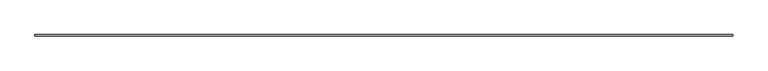
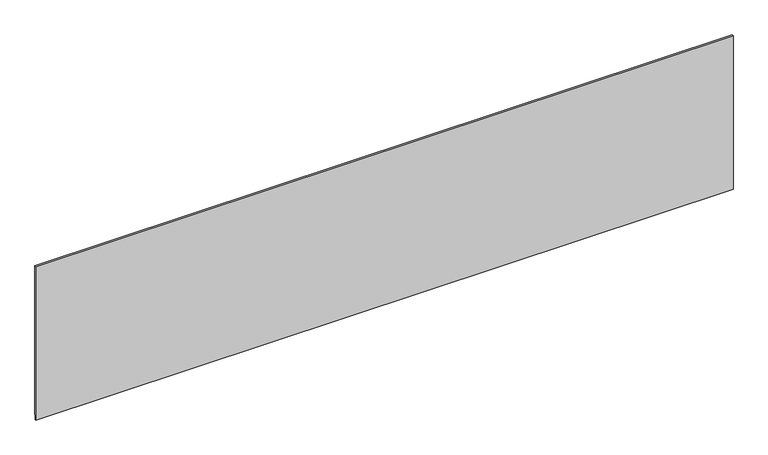
"""IFC4 building model written with IfcOpenShell, lengths in millimetres: proxy geometry, Generic Models 7:Generic Models 1:5:Generic Models 1:5 : Generic Models 7:Generic Models 1:337419:34 : Generic Models 7:Generic Models 1:5:Generic Models 1:5 : Generic Models 7:Generic Models 1:337419:311462."""

from ifc_helpers import new_model, si_unit, frame, origin, place, context, project, spatial, polyline, outline, extrude, source, transform, mapped, element, save


def generic_models_37c5037e(model_context):
    return source(origin(), model_context, "Body", "SweptSolid", [
        extrude(outline(polyline([(-579029.0720892, 3723.834699), (-579038.7913841, 3723.834699), (-579038.7913841, 6155.090949), (-579019.7413841, 6155.090949), (-579019.7413841, 3795.8780043), (-579029.0720892, 3784.758103), (-579029.0720892, 3723.834699)])), frame((793360.8632437, 0.0, 0.0), z_axis=(1.0, 0.0, 0.0), x_axis=(0.0, 1.0, 0.0)), (0.0, 0.0, 1.0), 10450.5125),
    ])


if __name__ == "__main__":
    model = new_model("IFC4")
    model_context = context("Model", 3, world=origin())
    ifc_project = project(units=[si_unit("LENGTHUNIT", "METRE", prefix="MILLI")], contexts=[model_context])
    site = spatial("IfcSite", under=ifc_project)
    building = spatial("IfcBuilding", under=site)
    placement = place(None, origin())
    generic_models_shape = generic_models_37c5037e(model_context)
    element("IfcBuildingElementProxy", 1, Name="Generic Models 7:Generic Models 1:5:Generic Models 1:5 : Generic Models 7:Generic Models 1:337419:34 : Generic Models 7:Generic Models 1:5:Generic Models 1:5 : Generic Models 7:Generic Models 1:337419:311462", ObjectType="Generic Models 7:Generic Models 1:5:Generic Models 1:5 : Generic Models 7:Generic Models 1:337419:34 : Generic Models 7:Generic Models 1:5:Generic Models 1:5 : Generic Models 7:Generic Models 1:337419:311462", at=placement, inside=building, context=model_context, shape_type="MappedRepresentation", body=[
        mapped(generic_models_shape, transform((0.0, 0.0, 0.0), x_axis=(1.0, 0.0, 0.0), y_axis=(0.0, 1.0, 0.0), z_axis=(0.0, 0.0, 1.0))),
    ])
    save(model, "model.ifc")

# Revit data of these elements
# Type "Generic Models 7:Generic Models 1:5:Generic Models 1:5 : Generic Models 7:Generic Models 1:337419:34 : Generic Models 7:Generic Models 1:5:Generic Models 1:5 : Generic Models 7:Generic Models 1:337419:311462"
#   NameOverride = "Generic Models 7:Generic Models 1:5:Generic Models 1:5 : Generic Models 7:Generic Models 1:337419:311462"
#   ObjectTypeOverride = "Generic Models 1:5 : Generic Models 7:Generic Models 1:337419"
#   Reference = "Generic Models 1"
#   Tag = "311462"
# Element 1 (IfcBuildingElementProxy, "Generic Models 7:Generic Models 1:5:Generic Models 1:5 : Generic Models 7:Generic Models 1:337419:34 : Generic Models 7:Generic Models 1:5:Generic Models 1:5 : Generic Models 7:Generic Models 1:337419:311462")
#   Materials on its faces: "1\" MINERAL WOOL BOARD INSULATION"
# Materials
#   "1\" MINERAL WOOL BOARD INSULATION": class "Unassigned", colour RGB 205 188 106, transparency 0, Cost = 0
